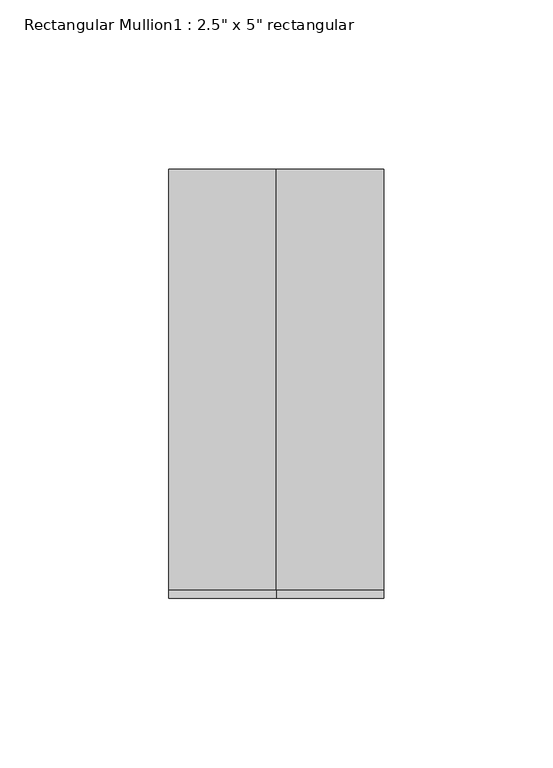
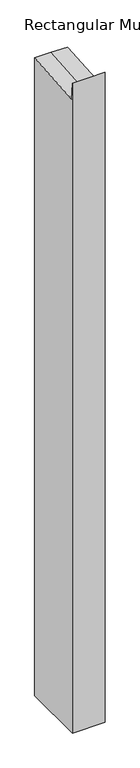
"""IFC4 building model written with IfcOpenShell, lengths in millimetres: member geometry."""

import ifcopenshell
import ifcopenshell.guid

model = None  # the IFC model being written
_history = None  # IfcOwnerHistory: only IFC2X3 demands one
_inside = {}  # id of a spatial element -> (the spatial element, [elements in it])
_under = {}  # id of a project, library or spatial element -> (it, [spatial elements below it])
_declared = {}  # id of a project -> (the project, [libraries it declares])
_typed = {}  # id of a type object -> (the type object, [elements of that type])
_made_of = {}  # id of a material, layer set ... -> (it, [elements and type objects made of it])


def new_model(schema):
    """Start an empty IFC model of exactly this schema.

    Asked for "IFC4X3", IfcOpenShell would pick the latest addendum, in which some entities
    have other attributes; the version numbers below select the first issue.
    IFC2X3 requires an IfcOwnerHistory on every rooted entity: one is made here for all.
    """
    global model, _history
    if schema == "IFC4X3":
        model = ifcopenshell.file(schema_version=(4, 3, 0, 0))
    else:
        model = ifcopenshell.file(schema=schema)
    _inside.clear()
    _under.clear()
    _declared.clear()
    _typed.clear()
    _made_of.clear()
    _history = None
    if model.schema == "IFC2X3":
        org = make("IfcOrganization", Name="unknown")
        user = make(
            "IfcPersonAndOrganization",
            ThePerson=make("IfcPerson", FamilyName="unknown"),
            TheOrganization=org,
        )
        app = make(
            "IfcApplication",
            ApplicationDeveloper=org,
            Version="unknown",
            ApplicationFullName="unknown",
            ApplicationIdentifier="unknown",
        )
        _history = make(
            "IfcOwnerHistory",
            OwningUser=user,
            OwningApplication=app,
            ChangeAction="ADDED",
            CreationDate=0,
        )
    return model


def make(cls, **values):
    """One entity of the class cls with the attributes given. An attribute that is None is left unset."""
    return model.create_entity(
        cls, **{name: value for name, value in values.items() if value is not None}
    )


def rooted(cls, **values):
    """An entity with a GlobalId (a new one), such as an element, a storey or a relation."""
    return make(cls, GlobalId=ifcopenshell.guid.new(), OwnerHistory=_history, **values)


def si_unit(unit_type, name, prefix=None):
    """IfcSIUnit, for example si_unit("LENGTHUNIT", "METRE", prefix="MILLI")."""
    return make("IfcSIUnit", UnitType=unit_type, Prefix=prefix, Name=name)


def assignment(units):
    """IfcUnitAssignment: the units of a project."""
    return None if units is None else make("IfcUnitAssignment", Units=units)


def point(xyz):
    """IfcCartesianPoint."""
    return None if xyz is None else make("IfcCartesianPoint", Coordinates=xyz)


def direction(xyz):
    """IfcDirection."""
    return None if xyz is None else make("IfcDirection", DirectionRatios=xyz)


def frame(location, z_axis=None, x_axis=None):
    """IfcAxis2Placement3D, a coordinate frame: its origin and axes. An axis left out is left unset."""
    return make(
        "IfcAxis2Placement3D",
        Location=point(location),
        Axis=direction(z_axis),
        RefDirection=direction(x_axis),
    )


def origin():
    """The frame at (0, 0, 0) with its axes left unset."""
    return frame((0.0, 0.0, 0.0))


def place(relative_to, where):
    """IfcLocalPlacement: puts the frame where relative to a parent placement (None: the world)."""
    return make(
        "IfcLocalPlacement", PlacementRelTo=relative_to, RelativePlacement=where
    )


def context(
    kind, dimensions, precision=None, world=None, true_north=None, identifier=None
):
    """IfcGeometricRepresentationContext, for example the 3D "Model" context."""
    return make(
        "IfcGeometricRepresentationContext",
        ContextIdentifier=identifier,
        ContextType=kind,
        CoordinateSpaceDimension=dimensions,
        Precision=precision,
        WorldCoordinateSystem=world,
        TrueNorth=true_north,
    )


def project(units=None, contexts=None):
    """IfcProject with its units and contexts."""
    return rooted(
        "IfcProject",
        Name="project",
        RepresentationContexts=contexts,
        UnitsInContext=assignment(units),
    )


def spatial(cls, under=None, at=None, **own):
    """A site, building, storey or space (cls), placed at a placement, below another one or the project."""
    s = rooted(cls, ObjectPlacement=at, **own)
    if under is not None:
        _under.setdefault(under.id(), (under, []))[1].append(s)
    return s


def faces_of(points, faces, orient=None, outer=None):
    """IfcFace entities. A face is a list of loops; a loop is a list of indices into points, from 0.

    orient and outer hold one flag for each loop. By default every Orientation is true, the
    first loop of a face is its IfcFaceOuterBound and the others are IfcFaceBound.
    """
    made = []
    for i, loops in enumerate(faces):
        bounds = []
        for j, loop in enumerate(loops):
            is_outer = j == 0 if outer is None else outer[i][j]
            bounds.append(
                make(
                    "IfcFaceOuterBound" if is_outer else "IfcFaceBound",
                    Bound=make("IfcPolyLoop", Polygon=[points[k] for k in loop]),
                    Orientation=True if orient is None else orient[i][j],
                )
            )
        made.append(make("IfcFace", Bounds=bounds))
    return made


def faceted_brep(points, faces, orient=None, outer=None, voids=None):
    """IfcFacetedBrep: a solid bounded by flat faces; with voids (closed shells), ...WithVoids."""
    shared = [point(p) for p in points]
    hull = make("IfcClosedShell", CfsFaces=faces_of(shared, faces, orient, outer))
    if voids is None:
        return make("IfcFacetedBrep", Outer=hull)
    return make(
        "IfcFacetedBrepWithVoids",
        Outer=hull,
        Voids=[
            make(cls, CfsFaces=faces_of(shared, fs, o, b)) for cls, fs, o, b in voids
        ],
    )


def shape(context_of_items, identifier, shape_type, items):
    """IfcShapeRepresentation: the items that make up one representation, for example the "Body"."""
    return make(
        "IfcShapeRepresentation",
        ContextOfItems=context_of_items,
        RepresentationIdentifier=identifier,
        RepresentationType=shape_type,
        Items=items,
    )


def source(mapping_origin, context_of_items, identifier, shape_type, items):
    """IfcRepresentationMap: a shape defined once, which mapped items show again and again."""
    return make(
        "IfcRepresentationMap",
        MappingOrigin=mapping_origin,
        MappedRepresentation=shape(context_of_items, identifier, shape_type, items),
    )


def transform(
    local_origin,
    x_axis=None,
    y_axis=None,
    z_axis=None,
    scale=None,
    scale2=None,
    scale3=None,
    uniform=True,
):
    """IfcCartesianTransformationOperator3D, or its non-uniform kind. x_axis, y_axis, z_axis: its Axis1, 2, 3."""
    if uniform:
        return make(
            "IfcCartesianTransformationOperator3D",
            Axis1=direction(x_axis),
            Axis2=direction(y_axis),
            LocalOrigin=point(local_origin),
            Scale=scale,
            Axis3=direction(z_axis),
        )
    return make(
        "IfcCartesianTransformationOperator3DnonUniform",
        Axis1=direction(x_axis),
        Axis2=direction(y_axis),
        LocalOrigin=point(local_origin),
        Scale=scale,
        Axis3=direction(z_axis),
        Scale2=scale2,
        Scale3=scale3,
    )


def mapped(mapping_source, mapping_target):
    """IfcMappedItem: shows the shape of a source again, moved by a transform."""
    return make(
        "IfcMappedItem", MappingSource=mapping_source, MappingTarget=mapping_target
    )


def made_of(thing, what):
    """Note that an element or type object is made of a material, layer set ...; save() writes the relation."""
    if what is not None:
        _made_of.setdefault(what.id(), (what, []))[1].append(thing)
    return thing


def element(
    cls,
    number,
    at=None,
    inside=None,
    cuts=None,
    type_object=None,
    material=None,
    context=None,
    identifier="Body",
    shape_type=None,
    held_by="IfcProductDefinitionShape",
    body=None,
    shapes=None,
    **own,
):
    """One element of the class cls, such as IfcWall. Its Tag is "e" and its number.

    at: its placement. inside: the storey or other place that contains it. cuts: it is an
    opening in that element (IfcRelVoidsElement). A single representation is given by context,
    identifier, shape_type and body (its items); several are given by shapes. held_by: the class
    of the entity that holds the representations. save() writes the other relations.
    """
    e = rooted(cls, Tag="e%d" % number, ObjectPlacement=at, **own)
    if body is not None:
        shapes = [shape(context, identifier, shape_type, body)]
    if shapes is not None:
        e.Representation = make(held_by, Representations=shapes)
    if inside is not None:
        _inside.setdefault(inside.id(), (inside, []))[1].append(e)
    if cuts is not None:
        rooted(
            "IfcRelVoidsElement", RelatingBuildingElement=cuts, RelatedOpeningElement=e
        )
    if type_object is not None:
        _typed.setdefault(type_object.id(), (type_object, []))[1].append(e)
    return made_of(e, material)


def aggregate(whole, parts):
    """IfcRelAggregates: a whole, such as a stair, and the parts it consists of."""
    return rooted("IfcRelAggregates", RelatingObject=whole, RelatedObjects=parts)


def save(model, path):
    """Write the relations noted so far, then the file.

    IfcRelAggregates (storeys below a building ...), IfcRelContainedInSpatialStructure (elements
    in a storey), IfcRelDefinesByType, IfcRelAssociatesMaterial and IfcRelDeclares: one each for
    every whole, place, type object, material and project.
    """
    for whole, parts in _under.values():
        aggregate(whole, parts)
    for where, things in _inside.values():
        rooted(
            "IfcRelContainedInSpatialStructure",
            RelatedElements=things,
            RelatingStructure=where,
        )
    for kind, things in _typed.values():
        rooted("IfcRelDefinesByType", RelatedObjects=things, RelatingType=kind)
    for what, things in _made_of.values():
        rooted("IfcRelAssociatesMaterial", RelatedObjects=things, RelatingMaterial=what)
    for by, libraries in _declared.values():
        rooted("IfcRelDeclares", RelatingContext=by, RelatedDefinitions=libraries)
    model.write(path)


def member_652a6926(model_context):
    return source(origin(), model_context, "Body", "Brep", [
        faceted_brep([(31.75, 63.5, -1302.7683735), (31.75, -63.5, -1302.7683735), (-31.75, -63.5, -1302.7683735), (-31.75, 63.5, -1302.7683735), (-31.75, 63.5, 4.512614), (0.0, 63.5, 4.512614), (31.75, 63.5, 4.512614), (-31.75, -63.5, 29.4551734), (-31.75, -61.0425175, -4.5008422), (31.75, -63.5, 29.4551734), (0.0, -63.5, 29.4551734), (31.75, -61.0425175, -4.5008422), (0.0, -61.0425175, -4.5008422)], [[[0, 1, 2, 3]], [[4, 5, 6, 0, 3]], [[7, 8, 4, 3, 2]], [[9, 10, 7, 2, 1]], [[6, 11, 9, 1, 0]], [[6, 5, 12, 11]], [[5, 4, 8, 12]], [[8, 7, 10, 12]], [[10, 9, 11, 12]]]),
    ])


if __name__ == "__main__":
    model = new_model("IFC4")
    model_context = context("Model", 3, world=origin())
    ifc_project = project(units=[si_unit("LENGTHUNIT", "METRE", prefix="MILLI")], contexts=[model_context])
    site = spatial("IfcSite", under=ifc_project)
    building = spatial("IfcBuilding", under=site)
    placement = place(None, origin())
    member_shape = member_652a6926(model_context)
    element("IfcMember", 1, ObjectType="Rectangular Mullion1 : 2.5\" x 5\" rectangular", at=placement, inside=building, context=model_context, shape_type="MappedRepresentation", body=[
        mapped(member_shape, transform((0.0, 0.0, 0.0), x_axis=(1.0, 0.0, 0.0), y_axis=(0.0, 1.0, 0.0), z_axis=(0.0, 0.0, 1.0))),
    ])
    save(model, "model.ifc")

# Revit data of these elements
# Type "Rectangular Mullion1 : 2.5\" x 5\" rectangular"
#   built-in parameter 1007304 = 0.416667 (stored number, unit not read)
#   built-in parameter 1007301 = 0.104167 (stored number, unit not read)
#   built-in parameter 1007300 = 0.104167 (stored number, unit not read)
# Element 1 (IfcMember, "Rectangular Mullion1 : 2.5\" x 5\" rectangular")
#   Materials on its faces: "support-frame"
# Materials
#   "support-frame": class "Unassigned", colour RGB 233 233 233, transparency 0, Cost = 0
